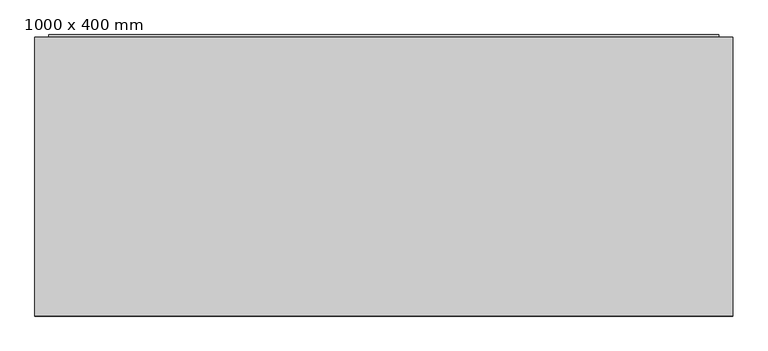
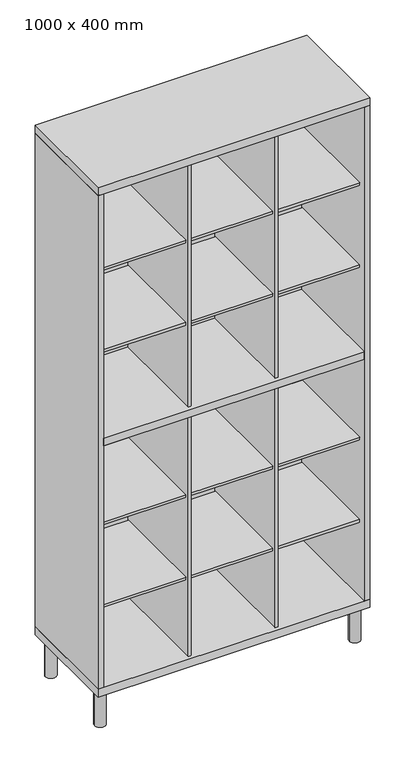
"""IFC4 building model written with IfcOpenShell, lengths in millimetres: furniture geometry, Módulo de estantería : 1000 x 400 mm."""

from ifc_helpers import new_model, si_unit, point, frame, frame_2d, origin, origin_with_axes, place, context, project, spatial, polyline, circle_curve, trimmed, segment, composite_curve, outline, extrude, source, transform, mapped, element, save


def furniture_1000_x_400_mm_99c9fea6(model_context):
    return source(origin(), model_context, "Body", "SweptSolid", [
        extrude(outline(polyline([(480.0, 191.424629), (-480.0, 191.424629), (-480.0, 194.424629), (480.0, 194.424629), (480.0, 191.424629)])), frame((0.0, 0.0, 170.0), z_axis=(0.0, 0.0, 1.0), x_axis=(1.0, 0.0, 0.0)), (0.0, 0.0, 1.0), 1920.0),
        extrude(outline(polyline([(-160.0, -180.0), (-470.0, -180.0), (-470.0, 186.2762655), (-160.0, 186.2762655), (-160.0, -180.0)])), frame((0.0, 0.0, 460.0), z_axis=(0.0, 0.0, 1.0), x_axis=(1.0, 0.0, 0.0)), (0.0, 0.0, 1.0), 10.0),
        extrude(outline(polyline([(160.0, -180.0), (-150.0, -180.0), (-150.0, 186.2762655), (160.0, 186.2762655), (160.0, -180.0)])), frame((0.0, 0.0, 460.0), z_axis=(0.0, 0.0, 1.0), x_axis=(1.0, 0.0, 0.0)), (0.0, 0.0, 1.0), 10.0),
        extrude(outline(polyline([(480.0, -180.0), (170.0, -180.0), (170.0, 186.2762655), (480.0, 186.2762655), (480.0, -180.0)])), frame((0.0, 0.0, 460.0), z_axis=(0.0, 0.0, 1.0), x_axis=(1.0, 0.0, 0.0)), (0.0, 0.0, 1.0), 10.0),
        extrude(outline(polyline([(-160.0, -180.0), (-470.0, -180.0), (-470.0, 186.2762655), (-160.0, 186.2762655), (-160.0, -180.0)])), frame((0.0, 0.0, 780.0), z_axis=(0.0, 0.0, 1.0), x_axis=(1.0, 0.0, 0.0)), (0.0, 0.0, 1.0), 10.0),
        extrude(outline(polyline([(160.0, -180.0), (-150.0, -180.0), (-150.0, 186.2762655), (160.0, 186.2762655), (160.0, -180.0)])), frame((0.0, 0.0, 780.0), z_axis=(0.0, 0.0, 1.0), x_axis=(1.0, 0.0, 0.0)), (0.0, 0.0, 1.0), 10.0),
        extrude(outline(polyline([(480.0, -180.0), (170.0, -180.0), (170.0, 186.2762655), (480.0, 186.2762655), (480.0, -180.0)])), frame((0.0, 0.0, 780.0), z_axis=(0.0, 0.0, 1.0), x_axis=(1.0, 0.0, 0.0)), (0.0, 0.0, 1.0), 10.0),
        extrude(outline(polyline([(-160.0, -180.0), (-470.0, -180.0), (-470.0, 186.2762655), (-160.0, 186.2762655), (-160.0, -180.0)])), frame((0.0, 0.0, 1450.0), z_axis=(0.0, 0.0, 1.0), x_axis=(1.0, 0.0, 0.0)), (0.0, 0.0, 1.0), 10.0),
        extrude(outline(polyline([(160.0, -180.0), (-150.0, -180.0), (-150.0, 186.2762655), (160.0, 186.2762655), (160.0, -180.0)])), frame((0.0, 0.0, 1450.0), z_axis=(0.0, 0.0, 1.0), x_axis=(1.0, 0.0, 0.0)), (0.0, 0.0, 1.0), 10.0),
        extrude(outline(polyline([(480.0, -180.0), (170.0, -180.0), (170.0, 186.2762655), (480.0, 186.2762655), (480.0, -180.0)])), frame((0.0, 0.0, 1450.0), z_axis=(0.0, 0.0, 1.0), x_axis=(1.0, 0.0, 0.0)), (0.0, 0.0, 1.0), 10.0),
        extrude(outline(polyline([(-160.0, -180.0), (-470.0, -180.0), (-470.0, 186.2762655), (-160.0, 186.2762655), (-160.0, -180.0)])), frame((0.0, 0.0, 1770.0), z_axis=(0.0, 0.0, 1.0), x_axis=(1.0, 0.0, 0.0)), (0.0, 0.0, 1.0), 10.0),
        extrude(outline(polyline([(160.0, -180.0), (-150.0, -180.0), (-150.0, 186.2762655), (160.0, 186.2762655), (160.0, -180.0)])), frame((0.0, 0.0, 1770.0), z_axis=(0.0, 0.0, 1.0), x_axis=(1.0, 0.0, 0.0)), (0.0, 0.0, 1.0), 10.0),
        extrude(outline(polyline([(480.0, -180.0), (170.0, -180.0), (170.0, 186.2762655), (480.0, 186.2762655), (480.0, -180.0)])), frame((0.0, 0.0, 1770.0), z_axis=(0.0, 0.0, 1.0), x_axis=(1.0, 0.0, 0.0)), (0.0, 0.0, 1.0), 10.0),
        extrude(outline(polyline([(170.0, -194.2277704), (160.0, -194.2277704), (160.0, 191.424629), (170.0, 191.424629), (170.0, -194.2277704)])), frame((0.0, 0.0, 170.0), z_axis=(0.0, 0.0, 1.0), x_axis=(1.0, 0.0, 0.0)), (0.0, 0.0, 1.0), 940.0),
        extrude(outline(polyline([(-150.0, -194.2277704), (-160.0, -194.2277704), (-160.0, 191.424629), (-150.0, 191.424629), (-150.0, -194.2277704)])), frame((0.0, 0.0, 170.0), z_axis=(0.0, 0.0, 1.0), x_axis=(1.0, 0.0, 0.0)), (0.0, 0.0, 1.0), 940.0),
        extrude(outline(polyline([(170.0, -194.2277704), (160.0, -194.2277704), (160.0, 191.424629), (170.0, 191.424629), (170.0, -194.2277704)])), frame((0.0, 0.0, 1140.0), z_axis=(0.0, 0.0, 1.0), x_axis=(1.0, 0.0, 0.0)), (0.0, 0.0, 1.0), 950.0),
        extrude(outline(polyline([(-150.0, -194.2277704), (-160.0, -194.2277704), (-160.0, 191.424629), (-150.0, 191.424629), (-150.0, -194.2277704)])), frame((0.0, 0.0, 1140.0), z_axis=(0.0, 0.0, 1.0), x_axis=(1.0, 0.0, 0.0)), (0.0, 0.0, 1.0), 950.0),
        extrude(outline(polyline([(480.0, -208.575371), (-480.0, -208.575371), (-480.0, 191.424629), (480.0, 191.424629), (480.0, -208.575371)])), frame((0.0, 0.0, 1110.0), z_axis=(0.0, 0.0, 1.0), x_axis=(1.0, 0.0, 0.0)), (0.0, 0.0, 1.0), 30.0),
        extrude(outline(composite_curve([segment(trimmed(circle_curve(frame_2d((-468.9411196, -166.8185459)), 20.0), [point((-448.9411196, -166.8185459))], [point((-488.9411196, -166.8185459))], False, "CARTESIAN"), True, "CONTINUOUS"), segment(trimmed(circle_curve(frame_2d((-468.9411196, -166.8185459)), 20.0), [point((-488.9411196, -166.8185459))], [point((-448.9411196, -166.8185459))], False, "CARTESIAN"), True, "CONTINUOUS")], self_intersect=False)), origin_with_axes(), (0.0, 0.0, 1.0), 140.0),
        extrude(outline(composite_curve([segment(trimmed(circle_curve(frame_2d((-468.9411196, 146.8185459)), 20.0), [point((-448.9411196, 146.8185459))], [point((-488.9411196, 146.8185459))], False, "CARTESIAN"), True, "CONTINUOUS"), segment(trimmed(circle_curve(frame_2d((-468.9411196, 146.8185459)), 20.0), [point((-488.9411196, 146.8185459))], [point((-448.9411196, 146.8185459))], False, "CARTESIAN"), True, "CONTINUOUS")], self_intersect=False)), origin_with_axes(), (0.0, 0.0, 1.0), 140.0),
        extrude(outline(composite_curve([segment(trimmed(circle_curve(frame_2d((468.9411196, -166.8185459)), 20.0), [point((448.9411196, -166.8185459))], [point((488.9411196, -166.8185459))], False, "CARTESIAN"), True, "CONTINUOUS"), segment(trimmed(circle_curve(frame_2d((468.9411196, -166.8185459)), 20.0), [point((488.9411196, -166.8185459))], [point((448.9411196, -166.8185459))], False, "CARTESIAN"), True, "CONTINUOUS")], self_intersect=False)), origin_with_axes(), (0.0, 0.0, 1.0), 140.0),
        extrude(outline(composite_curve([segment(trimmed(circle_curve(frame_2d((468.9411196, 146.8185459)), 20.0), [point((448.9411196, 146.8185459))], [point((488.9411196, 146.8185459))], False, "CARTESIAN"), True, "CONTINUOUS"), segment(trimmed(circle_curve(frame_2d((468.9411196, 146.8185459)), 20.0), [point((488.9411196, 146.8185459))], [point((448.9411196, 146.8185459))], False, "CARTESIAN"), True, "CONTINUOUS")], self_intersect=False)), origin_with_axes(), (0.0, 0.0, 1.0), 140.0),
        extrude(outline(polyline([(500.0, -208.575371), (-500.0, -208.575371), (-500.0, 191.424629), (500.0, 191.424629), (500.0, -208.575371)])), frame((0.0, 0.0, 2090.0), z_axis=(0.0, 0.0, 1.0), x_axis=(1.0, 0.0, 0.0)), (0.0, 0.0, 1.0), 30.0),
        extrude(outline(polyline([(500.0, -208.575371), (-500.0, -208.575371), (-500.0, 191.424629), (500.0, 191.424629), (500.0, -208.575371)])), frame((0.0, 0.0, 140.0), z_axis=(0.0, 0.0, 1.0), x_axis=(1.0, 0.0, 0.0)), (0.0, 0.0, 1.0), 30.0),
        extrude(outline(polyline([(-480.0, -208.575371), (-500.0, -208.575371), (-500.0, 191.424629), (-480.0, 191.424629), (-480.0, -208.575371)])), frame((0.0, 0.0, 170.0), z_axis=(0.0, 0.0, 1.0), x_axis=(1.0, 0.0, 0.0)), (0.0, 0.0, 1.0), 1920.0),
        extrude(outline(polyline([(500.0, -208.575371), (480.0, -208.575371), (480.0, 191.424629), (500.0, 191.424629), (500.0, -208.575371)])), frame((0.0, 0.0, 170.0), z_axis=(0.0, 0.0, 1.0), x_axis=(1.0, 0.0, 0.0)), (0.0, 0.0, 1.0), 1920.0),
    ])


if __name__ == "__main__":
    model = new_model("IFC4")
    model_context = context("Model", 3, world=origin())
    ifc_project = project(units=[si_unit("LENGTHUNIT", "METRE", prefix="MILLI")], contexts=[model_context])
    site = spatial("IfcSite", under=ifc_project)
    building = spatial("IfcBuilding", under=site)
    placement = place(None, origin())
    furniture_1000_x_400_mm_shape = furniture_1000_x_400_mm_99c9fea6(model_context)
    element("IfcFurniture", 1, ObjectType="Módulo de estantería : 1000 x 400 mm", at=placement, inside=building, context=model_context, shape_type="MappedRepresentation", body=[
        mapped(furniture_1000_x_400_mm_shape, transform((0.0, 0.0, 0.0), x_axis=(1.0, 0.0, 0.0), y_axis=(0.0, 1.0, 0.0), z_axis=(0.0, 0.0, 1.0))),
    ])
    save(model, "model.ifc")

# Revit data of these elements
# Type "Módulo de estantería : 1000 x 400 mm"
#   Máscara [instance default] = yes
#   Material de estructura = none
#   Material base = none
#   Material de estante = none
#   URL = ""
#   Model = ""
#   Default Elevation = 0
#   Description = (empty or 0)
#   Manufacturer = ""
#   Cost = 0
#   Assembly Code = ""
# Element 1 (IfcFurniture, "Módulo de estantería : 1000 x 400 mm")
#   Materials on its faces: "Madera - Listel"
# Materials
#   "Madera - Listel": class "Madera", colour RGB 210 180 110, transparency 0, Cost = 0
